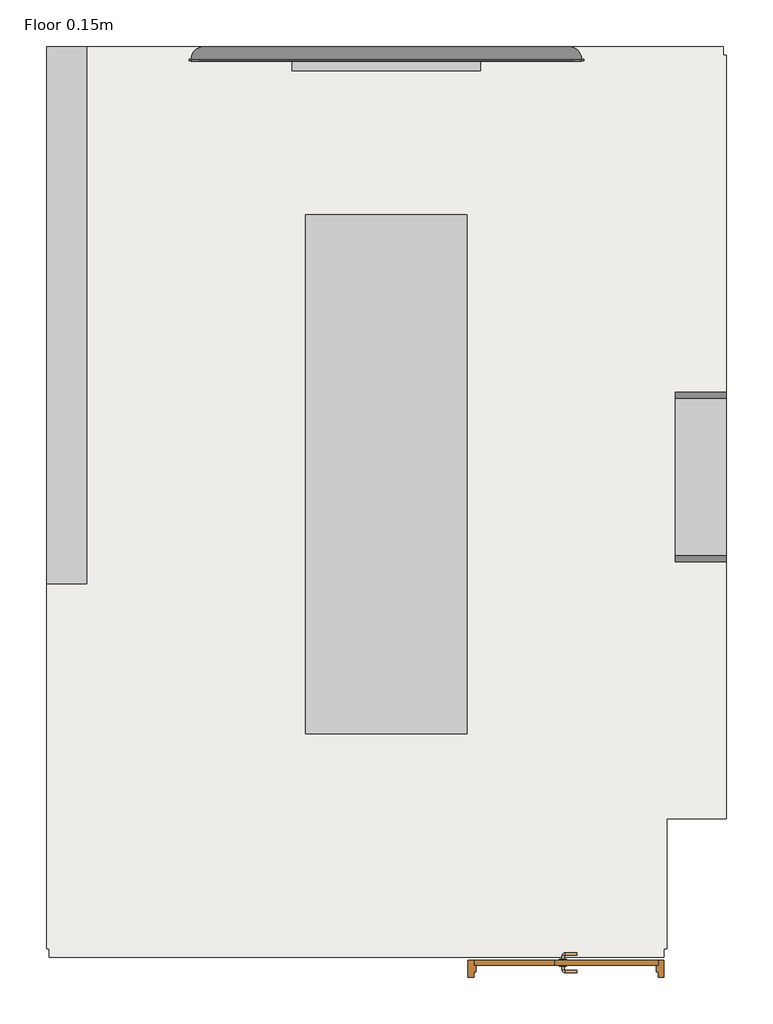
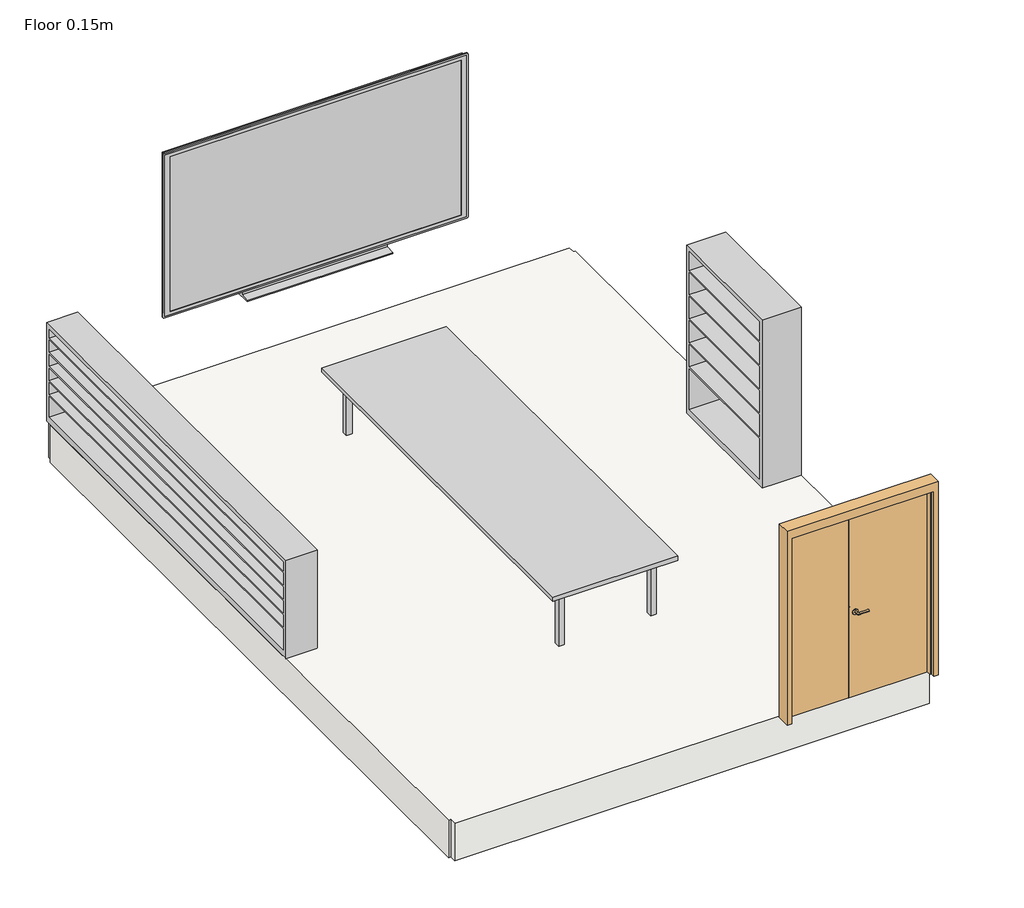
# One storey: 4 furniture elements, 1 door, 1 slab.
"""IFC4 building model written with IfcOpenShell, lengths in millimetres."""

import ifcopenshell
import ifcopenshell.guid

model = None  # the IFC model being written
_history = None  # IfcOwnerHistory: only IFC2X3 demands one
_inside = {}  # id of a spatial element -> (the spatial element, [elements in it])
_under = {}  # id of a project, library or spatial element -> (it, [spatial elements below it])
_declared = {}  # id of a project -> (the project, [libraries it declares])
_typed = {}  # id of a type object -> (the type object, [elements of that type])
_made_of = {}  # id of a material, layer set ... -> (it, [elements and type objects made of it])


def new_model(schema):
    """Start an empty IFC model of exactly this schema.

    Asked for "IFC4X3", IfcOpenShell would pick the latest addendum, in which some entities
    have other attributes; the version numbers below select the first issue.
    IFC2X3 requires an IfcOwnerHistory on every rooted entity: one is made here for all.
    """
    global model, _history
    if schema == "IFC4X3":
        model = ifcopenshell.file(schema_version=(4, 3, 0, 0))
    else:
        model = ifcopenshell.file(schema=schema)
    _inside.clear()
    _under.clear()
    _declared.clear()
    _typed.clear()
    _made_of.clear()
    _history = None
    if model.schema == "IFC2X3":
        org = make("IfcOrganization", Name="unknown")
        user = make(
            "IfcPersonAndOrganization",
            ThePerson=make("IfcPerson", FamilyName="unknown"),
            TheOrganization=org,
        )
        app = make(
            "IfcApplication",
            ApplicationDeveloper=org,
            Version="unknown",
            ApplicationFullName="unknown",
            ApplicationIdentifier="unknown",
        )
        _history = make(
            "IfcOwnerHistory",
            OwningUser=user,
            OwningApplication=app,
            ChangeAction="ADDED",
            CreationDate=0,
        )
    return model


def make(cls, **values):
    """One entity of the class cls with the attributes given. An attribute that is None is left unset."""
    return model.create_entity(
        cls, **{name: value for name, value in values.items() if value is not None}
    )


def rooted(cls, **values):
    """An entity with a GlobalId (a new one), such as an element, a storey or a relation."""
    return make(cls, GlobalId=ifcopenshell.guid.new(), OwnerHistory=_history, **values)


def si_unit(unit_type, name, prefix=None):
    """IfcSIUnit, for example si_unit("LENGTHUNIT", "METRE", prefix="MILLI")."""
    return make("IfcSIUnit", UnitType=unit_type, Prefix=prefix, Name=name)


def assignment(units):
    """IfcUnitAssignment: the units of a project."""
    return None if units is None else make("IfcUnitAssignment", Units=units)


def point(xyz):
    """IfcCartesianPoint."""
    return None if xyz is None else make("IfcCartesianPoint", Coordinates=xyz)


def direction(xyz):
    """IfcDirection."""
    return None if xyz is None else make("IfcDirection", DirectionRatios=xyz)


def frame(location, z_axis=None, x_axis=None):
    """IfcAxis2Placement3D, a coordinate frame: its origin and axes. An axis left out is left unset."""
    return make(
        "IfcAxis2Placement3D",
        Location=point(location),
        Axis=direction(z_axis),
        RefDirection=direction(x_axis),
    )


def frame_2d(location, x_axis=None):
    """IfcAxis2Placement2D, a coordinate frame in the plane: its origin and x axis."""
    return make(
        "IfcAxis2Placement2D", Location=point(location), RefDirection=direction(x_axis)
    )


def origin():
    """The frame at (0, 0, 0) with its axes left unset."""
    return frame((0.0, 0.0, 0.0))


def origin_with_axes():
    """The frame at (0, 0, 0) with the z axis (0, 0, 1) and the x axis (1, 0, 0) written out."""
    return frame((0.0, 0.0, 0.0), z_axis=(0.0, 0.0, 1.0), x_axis=(1.0, 0.0, 0.0))


def place(relative_to, where):
    """IfcLocalPlacement: puts the frame where relative to a parent placement (None: the world)."""
    return make(
        "IfcLocalPlacement", PlacementRelTo=relative_to, RelativePlacement=where
    )


def context(
    kind, dimensions, precision=None, world=None, true_north=None, identifier=None
):
    """IfcGeometricRepresentationContext, for example the 3D "Model" context."""
    return make(
        "IfcGeometricRepresentationContext",
        ContextIdentifier=identifier,
        ContextType=kind,
        CoordinateSpaceDimension=dimensions,
        Precision=precision,
        WorldCoordinateSystem=world,
        TrueNorth=true_north,
    )


def project(units=None, contexts=None):
    """IfcProject with its units and contexts."""
    return rooted(
        "IfcProject",
        Name="project",
        RepresentationContexts=contexts,
        UnitsInContext=assignment(units),
    )


def spatial(cls, under=None, at=None, **own):
    """A site, building, storey or space (cls), placed at a placement, below another one or the project."""
    s = rooted(cls, ObjectPlacement=at, **own)
    if under is not None:
        _under.setdefault(under.id(), (under, []))[1].append(s)
    return s


def polyline(points):
    """IfcPolyline through the points."""
    return make("IfcPolyline", Points=[point(p) for p in points])


def circle_curve(where, radius):
    """IfcCircle in the frame where."""
    return make("IfcCircle", Position=where, Radius=radius)


def ellipse_curve(where, semi_axis1, semi_axis2):
    """IfcEllipse in the frame where."""
    return make(
        "IfcEllipse", Position=where, SemiAxis1=semi_axis1, SemiAxis2=semi_axis2
    )


def trimmed(basis, trim1, trim2, sense, master):
    """IfcTrimmedCurve: the piece of a basis curve between two trims."""
    return make(
        "IfcTrimmedCurve",
        BasisCurve=basis,
        Trim1=trim1,
        Trim2=trim2,
        SenseAgreement=sense,
        MasterRepresentation=master,
    )


def segment(curve, same_sense, transition):
    """IfcCompositeCurveSegment."""
    return make(
        "IfcCompositeCurveSegment",
        Transition=transition,
        SameSense=same_sense,
        ParentCurve=curve,
    )


def composite_curve(segments, self_intersect=None):
    """IfcCompositeCurve: segments joined end to end."""
    return make("IfcCompositeCurve", Segments=segments, SelfIntersect=self_intersect)


def outline(outer, holes=None, kind="AREA"):
    """IfcArbitraryClosedProfileDef: a profile drawn as a closed curve; with holes, ...WithVoids."""
    if holes is None:
        return make("IfcArbitraryClosedProfileDef", ProfileType=kind, OuterCurve=outer)
    return make(
        "IfcArbitraryProfileDefWithVoids",
        ProfileType=kind,
        OuterCurve=outer,
        InnerCurves=holes,
    )


def extrude(swept, where, along, depth):
    """IfcExtrudedAreaSolid: the profile swept, set in the frame where, extruded along a direction by depth."""
    return make(
        "IfcExtrudedAreaSolid",
        SweptArea=swept,
        Position=where,
        ExtrudedDirection=direction(along),
        Depth=depth,
    )


def faces_of(points, faces, orient=None, outer=None):
    """IfcFace entities. A face is a list of loops; a loop is a list of indices into points, from 0.

    orient and outer hold one flag for each loop. By default every Orientation is true, the
    first loop of a face is its IfcFaceOuterBound and the others are IfcFaceBound.
    """
    made = []
    for i, loops in enumerate(faces):
        bounds = []
        for j, loop in enumerate(loops):
            is_outer = j == 0 if outer is None else outer[i][j]
            bounds.append(
                make(
                    "IfcFaceOuterBound" if is_outer else "IfcFaceBound",
                    Bound=make("IfcPolyLoop", Polygon=[points[k] for k in loop]),
                    Orientation=True if orient is None else orient[i][j],
                )
            )
        made.append(make("IfcFace", Bounds=bounds))
    return made


def faceted_brep(points, faces, orient=None, outer=None, voids=None):
    """IfcFacetedBrep: a solid bounded by flat faces; with voids (closed shells), ...WithVoids."""
    shared = [point(p) for p in points]
    hull = make("IfcClosedShell", CfsFaces=faces_of(shared, faces, orient, outer))
    if voids is None:
        return make("IfcFacetedBrep", Outer=hull)
    return make(
        "IfcFacetedBrepWithVoids",
        Outer=hull,
        Voids=[
            make(cls, CfsFaces=faces_of(shared, fs, o, b)) for cls, fs, o, b in voids
        ],
    )


def shape(context_of_items, identifier, shape_type, items):
    """IfcShapeRepresentation: the items that make up one representation, for example the "Body"."""
    return make(
        "IfcShapeRepresentation",
        ContextOfItems=context_of_items,
        RepresentationIdentifier=identifier,
        RepresentationType=shape_type,
        Items=items,
    )


def source(mapping_origin, context_of_items, identifier, shape_type, items):
    """IfcRepresentationMap: a shape defined once, which mapped items show again and again."""
    return make(
        "IfcRepresentationMap",
        MappingOrigin=mapping_origin,
        MappedRepresentation=shape(context_of_items, identifier, shape_type, items),
    )


def transform(
    local_origin,
    x_axis=None,
    y_axis=None,
    z_axis=None,
    scale=None,
    scale2=None,
    scale3=None,
    uniform=True,
):
    """IfcCartesianTransformationOperator3D, or its non-uniform kind. x_axis, y_axis, z_axis: its Axis1, 2, 3."""
    if uniform:
        return make(
            "IfcCartesianTransformationOperator3D",
            Axis1=direction(x_axis),
            Axis2=direction(y_axis),
            LocalOrigin=point(local_origin),
            Scale=scale,
            Axis3=direction(z_axis),
        )
    return make(
        "IfcCartesianTransformationOperator3DnonUniform",
        Axis1=direction(x_axis),
        Axis2=direction(y_axis),
        LocalOrigin=point(local_origin),
        Scale=scale,
        Axis3=direction(z_axis),
        Scale2=scale2,
        Scale3=scale3,
    )


def mapped(mapping_source, mapping_target):
    """IfcMappedItem: shows the shape of a source again, moved by a transform."""
    return make(
        "IfcMappedItem", MappingSource=mapping_source, MappingTarget=mapping_target
    )


def made_of(thing, what):
    """Note that an element or type object is made of a material, layer set ...; save() writes the relation."""
    if what is not None:
        _made_of.setdefault(what.id(), (what, []))[1].append(thing)
    return thing


def element(
    cls,
    number,
    at=None,
    inside=None,
    cuts=None,
    type_object=None,
    material=None,
    context=None,
    identifier="Body",
    shape_type=None,
    held_by="IfcProductDefinitionShape",
    body=None,
    shapes=None,
    **own,
):
    """One element of the class cls, such as IfcWall. Its Tag is "e" and its number.

    at: its placement. inside: the storey or other place that contains it. cuts: it is an
    opening in that element (IfcRelVoidsElement). A single representation is given by context,
    identifier, shape_type and body (its items); several are given by shapes. held_by: the class
    of the entity that holds the representations. save() writes the other relations.
    """
    e = rooted(cls, Tag="e%d" % number, ObjectPlacement=at, **own)
    if body is not None:
        shapes = [shape(context, identifier, shape_type, body)]
    if shapes is not None:
        e.Representation = make(held_by, Representations=shapes)
    if inside is not None:
        _inside.setdefault(inside.id(), (inside, []))[1].append(e)
    if cuts is not None:
        rooted(
            "IfcRelVoidsElement", RelatingBuildingElement=cuts, RelatedOpeningElement=e
        )
    if type_object is not None:
        _typed.setdefault(type_object.id(), (type_object, []))[1].append(e)
    return made_of(e, material)


def aggregate(whole, parts):
    """IfcRelAggregates: a whole, such as a stair, and the parts it consists of."""
    return rooted("IfcRelAggregates", RelatingObject=whole, RelatedObjects=parts)


def save(model, path):
    """Write the relations noted so far, then the file.

    IfcRelAggregates (storeys below a building ...), IfcRelContainedInSpatialStructure (elements
    in a storey), IfcRelDefinesByType, IfcRelAssociatesMaterial and IfcRelDeclares: one each for
    every whole, place, type object, material and project.
    """
    for whole, parts in _under.values():
        aggregate(whole, parts)
    for where, things in _inside.values():
        rooted(
            "IfcRelContainedInSpatialStructure",
            RelatedElements=things,
            RelatingStructure=where,
        )
    for kind, things in _typed.values():
        rooted("IfcRelDefinesByType", RelatedObjects=things, RelatingType=kind)
    for what, things in _made_of.values():
        rooted("IfcRelAssociatesMaterial", RelatedObjects=things, RelatingMaterial=what)
    for by, libraries in _declared.values():
        rooted("IfcRelDeclares", RelatingContext=by, RelatedDefinitions=libraries)
    model.write(path)


def plane_surface(at):
    """IfcPlane: the flat surface through the origin of the frame at, square to its z axis."""
    return make("IfcPlane", Position=at)


def cylinder_surface(at, radius):
    """IfcCylindricalSurface: all points at the distance radius from the z axis of the frame at."""
    return make("IfcCylindricalSurface", Position=at, Radius=radius)


def revolved_surface(curve, axis_point, axis_direction):
    """IfcSurfaceOfRevolution: the curve turned about the line through axis_point along axis_direction."""
    return make(
        "IfcSurfaceOfRevolution",
        SweptCurve=make("IfcArbitraryOpenProfileDef", ProfileType="CURVE", Curve=curve),
        AxisPosition=make("IfcAxis1Placement", Location=point(axis_point), Axis=direction(axis_direction)),
    )


def advanced_brep(points, edges, surfaces, faces):
    """IfcAdvancedBrep: a solid bounded by faces that lie on surfaces and meet in shared edges.

    An edge is (start, end): straight between two places in points (the first is 0);
    or (start, end, curve); or (start, end, curve, False) where it runs against its curve.
    A face is (place in surfaces, loops), or (place, loops, False) where it looks against
    its surface's normal. A loop lists edges by number (the first is 1), with a minus sign
    where the edge is run from its end to its start. The first loop is the outer one.
    """
    corners = [point(p) for p in points]
    vertices = [make("IfcVertexPoint", VertexGeometry=c) for c in corners]
    made = []
    for start, end, *more in edges:
        made.append(
            make(
                "IfcEdgeCurve",
                EdgeStart=vertices[start],
                EdgeEnd=vertices[end],
                EdgeGeometry=more[0] if more else make("IfcPolyline", Points=[corners[start], corners[end]]),
                SameSense=more[1] if len(more) > 1 else True,
            )
        )
    hull = []
    for where, loops, *sense in faces:
        bounds = []
        for j, loop in enumerate(loops):
            ring = [make("IfcOrientedEdge", EdgeElement=made[abs(k) - 1], Orientation=k > 0) for k in loop]
            bounds.append(
                make(
                    "IfcFaceOuterBound" if j == 0 else "IfcFaceBound",
                    Bound=make("IfcEdgeLoop", EdgeList=ring),
                    Orientation=True,
                )
            )
        hull.append(make("IfcAdvancedFace", Bounds=bounds, FaceSurface=surfaces[where], SameSense=sense[0] if sense else True))
    return make("IfcAdvancedBrep", Outer=make("IfcClosedShell", CfsFaces=hull))


def m_door_passage_uneven_flush_1600_x_2200_848efb9c(model_context):
    return source(origin(), model_context, "Body", "SolidModel", [
        advanced_brep(
        [(34.59375, 9.15, 1000.0), (14.59375, 9.15, 1000.0), (14.59375, 39.15, 1000.0), (34.59375, 39.15, 1000.0), (9.59375, 44.15, 1000.0), (9.59375, 64.15, 1000.0), (-95.40625, 64.15, 1000.0), (-95.40625, 44.15, 1000.0)],
        [
            (0, 1, circle_curve(frame((24.59375, 9.15, 1000.0), z_axis=(0.0, -1.0, 0.0), x_axis=(-1.0, 0.0, 0.0)), 10.0)),
            (1, 0, circle_curve(frame((24.59375, 9.15, 1000.0), z_axis=(0.0, -1.0, 0.0), x_axis=(-1.0, 0.0, 0.0)), 10.0)),
            (1, 2),
            (2, 3, circle_curve(frame((24.59375, 39.15, 1000.0), z_axis=(0.0, -1.0, 0.0), x_axis=(-1.0, 0.0, 0.0)), 10.0)),
            (3, 0),
            (3, 2, circle_curve(frame((24.59375, 39.15, 1000.0), z_axis=(0.0, -1.0, 0.0), x_axis=(-1.0, 0.0, 0.0)), 10.0)),
            (4, 5, circle_curve(frame((9.59375, 54.15, 1000.0), z_axis=(1.0, 0.0, 0.0), x_axis=(0.0, -1.0, 0.0)), 10.0)),
            (5, 3, circle_curve(frame((9.59375, 39.15, 1000.0), z_axis=(0.0, 0.0, -1.0), x_axis=(1.0, 0.0, 0.0)), 25.0)),
            (2, 4, circle_curve(frame((9.59375, 39.15, 1000.0), z_axis=(0.0, 0.0, 1.0), x_axis=(1.0, 0.0, 0.0)), 5.0)),
            (5, 4, circle_curve(frame((9.59375, 54.15, 1000.0), z_axis=(1.0, 0.0, 0.0), x_axis=(0.0, -1.0, 0.0)), 10.0)),
            (6, 7, circle_curve(frame((-95.40625, 54.15, 1000.0), z_axis=(-1.0, 0.0, 0.0), x_axis=(0.0, -1.0, 0.0)), 10.0)),
            (7, 6, circle_curve(frame((-95.40625, 54.15, 1000.0), z_axis=(-1.0, 0.0, 0.0), x_axis=(0.0, -1.0, 0.0)), 10.0)),
            (4, 7),
            (6, 5),
        ],
        [
            plane_surface(frame((24.59375, 9.15, 1000.0), z_axis=(0.0, -1.0, 0.0), x_axis=(0.0, 0.0, 1.0))),
            cylinder_surface(frame((24.59375, 9.15, 1000.0), z_axis=(0.0, -1.0, 0.0), x_axis=(-1.0, 0.0, 0.0)), 10.0),
            revolved_surface(trimmed(ellipse_curve(frame((24.59375, 39.15, 1000.0), z_axis=(0.0, 1.0, 0.0), x_axis=(-1.0, 0.0, 0.0)), 10.0, 10.0), [point((34.59375, 39.15, 1000.0))], [point((14.59375, 39.15, 1000.0))], True, "CARTESIAN"), (9.59375, 39.15, 1000.0), (0.0, 0.0, -1.0)),
            revolved_surface(trimmed(ellipse_curve(frame((24.59375, 39.15, 1000.0), z_axis=(0.0, 1.0, 0.0), x_axis=(-1.0, 0.0, 0.0)), 10.0, 10.0), [point((14.59375, 39.15, 1000.0))], [point((34.59375, 39.15, 1000.0))], True, "CARTESIAN"), (9.59375, 39.15, 1000.0), (0.0, 0.0, -1.0)),
            plane_surface(frame((-95.40625, 54.15, 1000.0), z_axis=(-1.0, 0.0, 0.0), x_axis=(0.0, 0.0, 1.0))),
            cylinder_surface(frame((9.59375, 54.15, 1000.0), z_axis=(1.0, 0.0, 0.0), x_axis=(0.0, -1.0, 0.0)), 10.0),
        ],
        [
            (0, [[1, 2]]),
            (1, [[3, 4, 5, -2]]),
            (1, [[-5, 6, -3, -1]]),
            (2, [[7, 8, -4, 9]]),
            (3, [[10, -9, -6, -8]]),
            (4, [[11, 12]]),
            (5, [[13, -11, 14, -7]]),
            (5, [[-14, -12, -13, -10]]),
        ],
    ),
        extrude(outline(composite_curve([segment(trimmed(circle_curve(frame_2d((1000.0, 27.09375)), 30.0), [point((1000.0, 57.09375))], [point((1000.0, -2.90625))], False, "CARTESIAN"), True, "CONTINUOUS"), segment(trimmed(circle_curve(frame_2d((1000.0, 27.09375)), 30.0), [point((1000.0, -2.90625))], [point((1000.0, 57.09375))], False, "CARTESIAN"), True, "CONTINUOUS")], self_intersect=False)), frame((0.0, 1.15, 0.0), z_axis=(0.0, 1.0, 0.0), x_axis=(0.0, 0.0, 1.0)), (0.0, 0.0, 1.0), 8.0),
        advanced_brep(
        [(34.59375, -51.85, 1000.0), (14.59375, -51.85, 1000.0), (34.59375, -81.85, 1000.0), (14.59375, -81.85, 1000.0), (9.59375, -86.85, 1000.0), (9.59375, -106.85, 1000.0), (-95.40625, -106.85, 1000.0), (-95.40625, -86.85, 1000.0)],
        [
            (0, 1, circle_curve(frame((24.59375, -51.85, 1000.0), z_axis=(0.0, 1.0, 0.0), x_axis=(-1.0, 0.0, 0.0)), 10.0)),
            (1, 0, circle_curve(frame((24.59375, -51.85, 1000.0), z_axis=(0.0, 1.0, 0.0), x_axis=(-1.0, 0.0, 0.0)), 10.0)),
            (0, 2),
            (2, 3, circle_curve(frame((24.59375, -81.85, 1000.0), z_axis=(0.0, 1.0, 0.0), x_axis=(-1.0, 0.0, 0.0)), 10.0)),
            (3, 1),
            (3, 2, circle_curve(frame((24.59375, -81.85, 1000.0), z_axis=(0.0, 1.0, 0.0), x_axis=(-1.0, 0.0, 0.0)), 10.0)),
            (4, 3, circle_curve(frame((9.59375, -81.85, 1000.0), z_axis=(0.0, 0.0, 1.0), x_axis=(1.0, 0.0, 0.0)), 5.0)),
            (2, 5, circle_curve(frame((9.59375, -81.85, 1000.0), z_axis=(0.0, 0.0, -1.0), x_axis=(1.0, 0.0, 0.0)), 25.0)),
            (5, 4, circle_curve(frame((9.59375, -96.85, 1000.0), z_axis=(1.0, 0.0, 0.0), x_axis=(0.0, 1.0, 0.0)), 10.0)),
            (4, 5, circle_curve(frame((9.59375, -96.85, 1000.0), z_axis=(1.0, 0.0, 0.0), x_axis=(0.0, 1.0, 0.0)), 10.0)),
            (6, 7, circle_curve(frame((-95.40625, -96.85, 1000.0), z_axis=(-1.0, 0.0, 0.0), x_axis=(0.0, 1.0, 0.0)), 10.0)),
            (7, 6, circle_curve(frame((-95.40625, -96.85, 1000.0), z_axis=(-1.0, 0.0, 0.0), x_axis=(0.0, 1.0, 0.0)), 10.0)),
            (5, 6),
            (7, 4),
        ],
        [
            plane_surface(frame((24.59375, -51.85, 1000.0), z_axis=(0.0, 1.0, 0.0), x_axis=(0.0, 0.0, 1.0))),
            cylinder_surface(frame((24.59375, -51.85, 1000.0), z_axis=(0.0, 1.0, 0.0), x_axis=(-1.0, 0.0, 0.0)), 10.0),
            revolved_surface(trimmed(ellipse_curve(frame((24.59375, -81.85, 1000.0), z_axis=(0.0, 1.0, 0.0), x_axis=(-1.0, 0.0, 0.0)), 10.0, 10.0), [point((34.59375, -81.85, 1000.0))], [point((14.59375, -81.85, 1000.0))], True, "CARTESIAN"), (9.59375, -81.85, 1000.0), (0.0, 0.0, -1.0)),
            revolved_surface(trimmed(ellipse_curve(frame((24.59375, -81.85, 1000.0), z_axis=(0.0, 1.0, 0.0), x_axis=(-1.0, 0.0, 0.0)), 10.0, 10.0), [point((14.59375, -81.85, 1000.0))], [point((34.59375, -81.85, 1000.0))], True, "CARTESIAN"), (9.59375, -81.85, 1000.0), (0.0, 0.0, -1.0)),
            plane_surface(frame((-95.40625, -96.85, 1000.0), z_axis=(-1.0, 0.0, 0.0), x_axis=(0.0, 0.0, 1.0))),
            cylinder_surface(frame((9.59375, -96.85, 1000.0), z_axis=(1.0, 0.0, 0.0), x_axis=(0.0, 1.0, 0.0)), 10.0),
        ],
        [
            (0, [[1, 2]]),
            (1, [[-1, 3, 4, 5]]),
            (1, [[-2, -5, 6, -3]]),
            (2, [[7, -4, 8, 9]]),
            (3, [[-8, -6, -7, 10]]),
            (4, [[11, 12]]),
            (5, [[-9, 13, -12, 14]]),
            (5, [[-10, -14, -11, -13]]),
        ],
    ),
        extrude(outline(composite_curve([segment(trimmed(circle_curve(frame_2d((1000.0, 27.09375)), 30.0), [point((1000.0, 57.09375))], [point((1000.0, -2.90625))], False, "CARTESIAN"), True, "CONTINUOUS"), segment(trimmed(circle_curve(frame_2d((1000.0, 27.09375)), 30.0), [point((1000.0, -2.90625))], [point((1000.0, 57.09375))], False, "CARTESIAN"), True, "CONTINUOUS")], self_intersect=False)), frame((0.0, -51.85, 0.0), z_axis=(0.0, 1.0, 0.0), x_axis=(0.0, 0.0, 1.0)), (0.0, 0.0, 1.0), 8.0),
        extrude(outline(polyline([(98.4, 1.15), (98.4, -43.85), (-800.0, -43.85), (-800.0, 1.15), (98.4, 1.15)])), origin_with_axes(), (0.0, 0.0, 1.0), 2200.0),
        faceted_brep([(800.0, 5.9125, 0.0), (784.125, 5.9125, 0.0), (784.125, 56.9375, 0.0), (800.0, 56.9375, 0.0), (800.0, 106.15, 0.0), (850.0, 106.15, 0.0), (850.0, -43.85, 0.0), (800.0, -43.85, 0.0), (800.0, -43.85, 2200.0), (800.0, 5.9125, 2200.0), (850.0, -43.85, 2300.0), (-850.0, -43.85, 2300.0), (-850.0, -43.85, 0.0), (-800.0, -43.85, 0.0), (-800.0, -43.85, 2200.0), (850.0, 106.15, 2300.0), (800.0, 106.15, 2200.0), (-800.0, 106.15, 2200.0), (-800.0, 106.15, 0.0), (-850.0, 106.15, 0.0), (-850.0, 106.15, 2300.0), (800.0, 56.9375, 2200.0), (784.125, 56.9375, 2184.125), (-784.125, 56.9375, 2184.125), (-784.125, 56.9375, 0.0), (-800.0, 56.9375, 0.0), (-800.0, 56.9375, 2200.0), (784.125, 5.9125, 2184.125), (-800.0, 5.9125, 2200.0), (-800.0, 5.9125, 0.0), (-784.125, 5.9125, 0.0), (-784.125, 5.9125, 2184.125)], [[[0, 1, 2, 3, 4, 5, 6, 7]], [[7, 8, 9, 0]], [[6, 10, 11, 12, 13, 14, 8, 7]], [[5, 15, 10, 6]], [[4, 16, 17, 18, 19, 20, 15, 5]], [[3, 21, 16, 4]], [[2, 22, 23, 24, 25, 26, 21, 3]], [[1, 27, 22, 2]], [[0, 9, 28, 29, 30, 31, 27, 1]], [[8, 14, 28, 9]], [[16, 21, 26, 17]], [[22, 27, 31, 23]], [[12, 19, 18, 25, 24, 30, 29, 13]], [[13, 29, 28, 14]], [[11, 20, 19, 12]], [[17, 26, 25, 18]], [[23, 31, 30, 24]], [[15, 20, 11, 10]]]),
        extrude(outline(polyline([(800.0, 1.15), (800.0, -43.85), (101.6, -43.85), (101.6, 1.15), (800.0, 1.15)])), origin_with_axes(), (0.0, 0.0, 1.0), 2200.0),
    ])


def furniture_0810mm_1eea789d(model_context):
    return source(origin(), model_context, "Body", "SolidModel", [
        advanced_brep(
        [(-1698.1126034, -51.4613764, 80.0), (1690.2235751, -51.4613764, 80.0), (1690.2235751, -51.4613764, 1998.6077952), (-1698.1126034, -51.4613764, 1998.6077952), (1580.2235751, 58.5386236, 80.0), (-1588.1126034, 58.5386236, 80.0), (-1588.1126034, 58.5386236, 1888.6077952), (1580.2235751, 58.5386236, 1888.6077952)],
        [
            (0, 1),
            (1, 2),
            (2, 3),
            (3, 0),
            (4, 5),
            (5, 6),
            (6, 7),
            (7, 4),
            (0, 5, circle_curve(frame((-1588.1126034, -51.4613764, 80.0), z_axis=(0.0, 0.0, -1.0), x_axis=(-1.0, 0.0, 0.0)), 110.0)),
            (4, 1, circle_curve(frame((1580.2235751, -51.4613764, 80.0), z_axis=(0.0, 0.0, -1.0), x_axis=(1.0, 0.0, 0.0)), 110.0)),
            (7, 2, ellipse_curve(frame((1580.2235751, -51.4613764, 1888.6077952), z_axis=(0.7071067811865475, 0.0, -0.7071067811865475), x_axis=(0.7071067811865474, 0.0, 0.7071067811865476)), 155.5634919, 110.0)),
            (6, 3, ellipse_curve(frame((-1588.1126034, -51.4613764, 1888.6077952), z_axis=(0.7071067811865475, 0.0, 0.7071067811865475), x_axis=(-0.7071067811865476, 0.0, 0.7071067811865474)), 155.5634919, 110.0)),
        ],
        [
            plane_surface(frame((-1698.1126034, -51.4613764, 1998.6077952), z_axis=(0.0, -1.0, 0.0), x_axis=(-1.0, 0.0, 0.0))),
            plane_surface(frame((-1698.1126034, 58.5386236, 1998.6077952), z_axis=(0.0, 1.0, 0.0), x_axis=(1.0, 0.0, 0.0))),
            plane_surface(frame((-1698.1126034, -51.4613764, 80.0), z_axis=(0.0, 0.0, -1.0), x_axis=(0.0, 1.0, 0.0))),
            cylinder_surface(frame((1580.2235751, -51.4613764, 80.0), z_axis=(0.0, 0.0, 1.0), x_axis=(1.0, 0.0, 0.0)), 110.0),
            cylinder_surface(frame((1690.2235751, -51.4613764, 1888.6077952), z_axis=(-1.0, 0.0, 0.0), x_axis=(0.0, 0.0, 1.0)), 110.0),
            cylinder_surface(frame((-1588.1126034, -51.4613764, 1998.6077952), z_axis=(0.0, 0.0, -1.0), x_axis=(-1.0, 0.0, 0.0)), 110.0),
        ],
        [
            (0, [[1, 2, 3, 4]]),
            (1, [[5, 6, 7, 8]]),
            (2, [[-1, 9, -5, 10]]),
            (3, [[11, -2, -10, -8]]),
            (4, [[-11, -7, 12, -3]]),
            (5, [[-12, -6, -9, -4]]),
        ],
    ),
        extrude(outline(composite_curve([segment(polyline([(2018.6077952, 1695.2235751), (2018.6077952, -1703.1126034)]), True, "CONTINUOUS"), segment(trimmed(circle_curve(frame_2d((2003.6077952, -1703.1126034)), 15.0), [point((2018.6077952, -1703.1126034))], [point((2003.6077952, -1718.1126034))], False, "CARTESIAN"), True, "CONTINUOUS"), segment(polyline([(2003.6077952, -1718.1126034), (75.0, -1718.1126034)]), True, "CONTINUOUS"), segment(trimmed(circle_curve(frame_2d((75.0, -1703.1126034)), 15.0), [point((75.0, -1718.1126034))], [point((60.0, -1703.1126034))], False, "CARTESIAN"), True, "CONTINUOUS"), segment(polyline([(60.0, -1703.1126034), (60.0, 1695.2235751)]), True, "CONTINUOUS"), segment(trimmed(circle_curve(frame_2d((75.0, 1695.2235751)), 15.0), [point((60.0, 1695.2235751))], [point((75.0, 1710.2235751))], False, "CARTESIAN"), True, "CONTINUOUS"), segment(polyline([(75.0, 1710.2235751), (2003.6077952, 1710.2235751)]), True, "CONTINUOUS"), segment(trimmed(circle_curve(frame_2d((2003.6077952, 1695.2235751)), 15.0), [point((2003.6077952, 1710.2235751))], [point((2018.6077952, 1695.2235751))], False, "CARTESIAN"), True, "CONTINUOUS")], self_intersect=False), holes=[polyline([(1998.6077952, 1690.2235751), (80.0, 1690.2235751), (80.0, -1698.1126034), (1998.6077952, -1698.1126034), (1998.6077952, 1690.2235751)])]), frame((0.0, -66.4613764, 0.0), z_axis=(0.0, 1.0, 0.0), x_axis=(0.0, 0.0, 1.0)), (0.0, 0.0, 1.0), 15.0),
        faceted_brep([(1690.2235751, -69.4613764, 1998.6077952), (-1698.1126034, -69.4613764, 1998.6077952), (-1698.1126034, -69.4613764, 80.0), (1690.2235751, -69.4613764, 80.0), (-1638.1126034, -69.4613764, 1958.6077952), (1630.2235751, -69.4613764, 1958.6077952), (1630.2235751, -69.4613764, 120.0), (-1638.1126034, -69.4613764, 120.0), (1690.2235751, -51.4613764, 1998.6077952), (1690.2235751, -51.4613764, 80.0), (-1698.1126034, -51.4613764, 80.0), (-1698.1126034, -51.4613764, 1998.6077952), (-1638.1126034, -66.4613764, 1958.6077952), (-1638.1126034, -66.4613764, 120.0), (1630.2235751, -66.4613764, 120.0), (1630.2235751, -66.4613764, 1958.6077952)], [[[0, 1, 2, 3], [4, 5, 6, 7]], [[8, 9, 10, 11]], [[1, 0, 8, 11]], [[2, 1, 11, 10]], [[3, 2, 10, 9]], [[0, 3, 9, 8]], [[12, 13, 14, 15]], [[12, 15, 5, 4]], [[15, 14, 6, 5]], [[14, 13, 7, 6]], [[13, 12, 4, 7]]]),
        extrude(outline(polyline([(-51.4613764, 80.0), (-1.4613764, 80.0), (48.5386236, 0.0), (-151.4613764, 0.0), (-151.4613764, 10.0), (-51.4613764, 20.0), (-51.4613764, 80.0)])), frame((-821.0285588, 0.0, 0.0), z_axis=(1.0, 0.0, 0.0), x_axis=(0.0, 1.0, 0.0)), (0.0, 0.0, 1.0), 1634.1680892),
    ])


def m_shelving_left_2_f9164daf(model_context):
    return source(origin(), model_context, "Body", "SweptSolid", [
        extrude(outline(polyline([(0.0, 2330.0), (1170.0, 2330.0), (1170.0, -2330.0), (0.0, -2330.0), (0.0, 2330.0)]), holes=[polyline([(1119.2, 2279.2), (1015.5571429, 2279.2), (1015.5571429, -2279.2), (1119.2, -2279.2), (1119.2, 2279.2)]), polyline([(76.2, 2279.2), (76.2, -2279.2), (321.5857143, -2279.2), (321.5857143, 2279.2), (76.2, 2279.2)]), polyline([(681.2714286, -2279.2), (823.0142857, -2279.2), (823.0142857, 2279.2), (681.2714286, 2279.2), (681.2714286, -2279.2)]), polyline([(990.1571429, 2279.2), (848.4142857, 2279.2), (848.4142857, -2279.2), (990.1571429, -2279.2), (990.1571429, 2279.2)]), polyline([(655.8714286, 2279.2), (514.1285714, 2279.2), (514.1285714, -2279.2), (655.8714286, -2279.2), (655.8714286, 2279.2)]), polyline([(488.7285714, 2279.2), (346.9857143, 2279.2), (346.9857143, -2279.2), (488.7285714, -2279.2), (488.7285714, 2279.2)])]), frame((0.0, -479.8, 0.0), z_axis=(0.0, 1.0, 0.0), x_axis=(0.0, 0.0, 1.0)), (0.0, 0.0, 1.0), 350.0),
    ])


def m_shelving_right_232c7dd4(model_context):
    return source(origin(), model_context, "Body", "SweptSolid", [
        extrude(outline(polyline([(0.0, 735.0), (2000.0, 735.0), (2000.0, -735.0), (0.0, -735.0), (0.0, 735.0)]), holes=[polyline([(1949.2, 684.2), (1726.9857143, 684.2), (1726.9857143, -684.2), (1949.2, -684.2), (1949.2, 684.2)]), polyline([(76.2, 684.2), (76.2, -684.2), (558.7285714, -684.2), (558.7285714, 684.2), (76.2, 684.2)]), polyline([(1155.5571429, -684.2), (1415.8714286, -684.2), (1415.8714286, 684.2), (1155.5571429, 684.2), (1155.5571429, -684.2)]), polyline([(1701.5857143, 684.2), (1441.2714286, 684.2), (1441.2714286, -684.2), (1701.5857143, -684.2), (1701.5857143, 684.2)]), polyline([(1130.1571429, 684.2), (869.8428571, 684.2), (869.8428571, -684.2), (1130.1571429, -684.2), (1130.1571429, 684.2)]), polyline([(844.4428571, 684.2), (584.1285714, 684.2), (584.1285714, -684.2), (844.4428571, -684.2), (844.4428571, 684.2)])]), frame((0.0, -524.8, 0.0), z_axis=(0.0, 1.0, 0.0), x_axis=(0.0, 0.0, 1.0)), (0.0, 0.0, 1.0), 440.0),
    ])


def m_table_rectangular_table_5a2d8c47(model_context):
    return source(origin(), model_context, "Body", "SweptSolid", [
        extrude(outline(polyline([(-2034.1, 547.6), (-2034.1, 484.1), (-2097.6, 484.1), (-2097.6, 547.6), (-2034.1, 547.6)])), origin_with_axes(), (0.0, 0.0, 1.0), 679.2),
        extrude(outline(polyline([(2034.1, 547.6), (2097.6, 547.6), (2097.6, 484.1), (2034.1, 484.1), (2034.1, 547.6)])), origin_with_axes(), (0.0, 0.0, 1.0), 679.2),
        extrude(outline(polyline([(-2034.1, -547.6), (-2097.6, -547.6), (-2097.6, -484.1), (-2034.1, -484.1), (-2034.1, -547.6)])), origin_with_axes(), (0.0, 0.0, 1.0), 679.2),
        extrude(outline(polyline([(2034.1, -547.6), (2034.1, -484.1), (2097.6, -484.1), (2097.6, -547.6), (2034.1, -547.6)])), origin_with_axes(), (0.0, 0.0, 1.0), 679.2),
        extrude(outline(polyline([(2250.0, 700.0), (2250.0, -700.0), (-2250.0, -700.0), (-2250.0, 700.0), (2250.0, 700.0)])), frame((0.0, 0.0, 679.2), z_axis=(0.0, 0.0, 1.0), x_axis=(1.0, 0.0, 0.0)), (0.0, 0.0, 1.0), 50.8),
        extrude(outline(polyline([(2034.1, 509.5), (2034.1, 484.1), (-2034.1, 484.1), (-2034.1, 509.5), (2034.1, 509.5)])), frame((0.0, 0.0, 577.6), z_axis=(0.0, 0.0, 1.0), x_axis=(1.0, 0.0, 0.0)), (0.0, 0.0, 1.0), 101.6),
        extrude(outline(polyline([(2034.1, -509.5), (-2034.1, -509.5), (-2034.1, -484.1), (2034.1, -484.1), (2034.1, -509.5)])), frame((0.0, 0.0, 577.6), z_axis=(0.0, 0.0, 1.0), x_axis=(1.0, 0.0, 0.0)), (0.0, 0.0, 1.0), 101.6),
        extrude(outline(polyline([(-2046.8, -484.1), (-2072.2, -484.1), (-2072.2, 484.1), (-2046.8, 484.1), (-2046.8, -484.1)])), frame((0.0, 0.0, 577.6), z_axis=(0.0, 0.0, 1.0), x_axis=(1.0, 0.0, 0.0)), (0.0, 0.0, 1.0), 101.6),
        extrude(outline(polyline([(2046.8, -484.1), (2046.8, 484.1), (2072.2, 484.1), (2072.2, -484.1), (2046.8, -484.1)])), frame((0.0, 0.0, 577.6), z_axis=(0.0, 0.0, 1.0), x_axis=(1.0, 0.0, 0.0)), (0.0, 0.0, 1.0), 101.6),
    ])


model = new_model("IFC4")

# Units and contexts
model_context = context("Model", 3, world=origin())
ifc_project = project(units=[si_unit("LENGTHUNIT", "METRE", prefix="MILLI")], contexts=[model_context])

# Site, building, storey
site = spatial("IfcSite", under=ifc_project)
building = spatial("IfcBuilding", under=site)
storey = spatial("IfcBuildingStorey", under=building, Name="Floor 0.15m", Elevation=150.0)

# Door
placement = place(None, origin())
m_door_passage_uneven_flush_1600_x_2200_shape = m_door_passage_uneven_flush_1600_x_2200_848efb9c(model_context)
element("IfcDoor", 1, ObjectType="M_Door-Passage-Uneven-Flush : 1600 X 2200", at=placement, inside=storey, context=model_context, shape_type="MappedRepresentation", body=[
    mapped(m_door_passage_uneven_flush_1600_x_2200_shape, transform((1406.2835652, -4036.1029692, 150.0), x_axis=(-1.0, 0.0, 0.0), y_axis=(0.0, -1.0, 0.0), z_axis=(0.0, 0.0, 1.0))),
])

# Furniture
furniture_0810mm_shape = furniture_0810mm_1eea789d(model_context)
element("IfcFurniture", 2, ObjectType="M_TV - Flat Screen : 0810mm", at=placement, inside=storey, context=model_context, shape_type="MappedRepresentation", body=[
    mapped(furniture_0810mm_shape, transform((-149.7719206, 3874.2084071, 950.0), x_axis=(1.0, 0.0, 0.0), y_axis=(0.0, 1.0, 0.0), z_axis=(0.0, 0.0, 1.0))),
])
m_shelving_left_2_shape = m_shelving_left_2_f9164daf(model_context)
element("IfcFurniture", 3, ObjectType="M_Shelving : LEFT_2", at=placement, inside=storey, context=model_context, shape_type="MappedRepresentation", body=[
    mapped(m_shelving_left_2_shape, transform((-3233.5164348, 1602.7470308, 150.0), x_axis=(0.0, 1.0, 0.0), y_axis=(-1.0, 0.0, 0.0), z_axis=(0.0, 0.0, 1.0))),
])
m_shelving_right_shape = m_shelving_right_232c7dd4(model_context)
element("IfcFurniture", 4, ObjectType="M_Shelving : RIGHT", at=placement, inside=storey, context=model_context, shape_type="MappedRepresentation", body=[
    mapped(m_shelving_right_shape, transform((2271.4835652, 197.7470308, 150.0), x_axis=(0.0, 1.0, 0.0), y_axis=(-1.0, 0.0, 0.0), z_axis=(0.0, 0.0, 1.0))),
])
m_table_rectangular_table_shape = m_table_rectangular_table_5a2d8c47(model_context)
element("IfcFurniture", 5, ObjectType="M_Table-Rectangular : TABLE", at=placement, inside=storey, context=model_context, shape_type="MappedRepresentation", body=[
    mapped(m_table_rectangular_table_shape, transform((-153.7164348, 222.7470308, 150.0), x_axis=(0.0, 1.0, 0.0), y_axis=(-1.0, 0.0, 0.0), z_axis=(0.0, 0.0, 1.0))),
])

# Slab
element("IfcSlab", 6, ObjectType="FLOOR", at=placement, inside=storey, context=model_context, shape_type="SweptSolid", body=[
    extrude(outline(polyline([(-3078.7164348, -3892.2529692), (-3103.7164348, -3892.2529692), (-3103.7164348, 3857.7470308), (-3078.7164348, 3857.7470308), (-3078.7164348, 3932.7470308), (2771.2835652, 3932.7470308), (2771.2835652, 3857.7470308), (2796.2835652, 3857.7470308), (2796.2835652, -2767.2529692), (2281.2835652, -2767.2529692), (2281.2835652, -3892.2529692), (2256.2835652, -3892.2529692), (2256.2835652, -3967.2529692), (-3078.7164348, -3967.2529692), (-3078.7164348, -3892.2529692)])), frame((0.0, 0.0, -295.0), z_axis=(0.0, 0.0, 1.0), x_axis=(1.0, 0.0, 0.0)), (0.0, 0.0, 1.0), 445.0),
])

save(model, "model.ifc")

# Revit data of these elements
# Type "M_Door-Passage-Uneven-Flush : 1600 X 2200"
#   Type Mark = "50"
#   Assembly Code = "C1020300"
#   Analytic Construction = "Wooden"
#   Width Large Panel = 900 mm
#   W = 700 mm
#   Thickness = 45 mm
#   Thermal Resistance (R) = 0.455703 (m²·K)/W
#   Swing Angle [instance default] = 90.00°
#   Strike Height = 1000 mm
#   Rough Width [instance default] = 1700 mm
#   Rough Height [instance default] = 2300 mm
#   Masonry Frame Opening Height [instance default] = 100 mm
#   Masonry Frame Opening Width [instance default] = 100 mm
#   Inset Calculation [instance default] = 105 mm
#   Masonry Inset [instance default] = 25 mm
#   Height = 2200 mm
#   Width = 1600 mm
#   Heat Transfer Coefficient (U) = 2.19465 W/(m²·K)
#   Masonry Frame Depth = 150 mm
#   Masonry Frame [instance default] = yes
#   Dry Wall Frame [instance default] = no
#   Panel Material = Wood - Birch
#   Frame Material = Metal - Paint Finish - Grey
#   Door Handle Material = Aluminum
#   Visual Light Transmittance = 0
#   Solar Heat Gain Coefficient = 0
#   Wall Closure = (empty or 0)
#   Function = (empty or 0)
# Type "M_TV - Flat Screen : 0810mm"
#   SinAng = 0.49 mm
#   L = 3268.336 mm
#   H = 1838.608 mm
#   Thickness = 110 mm
#   Diagonal = 3750 mm
#   CosAng = 0.872 mm
#   Stand [instance default] = yes
#   Default Elevation = 0
# Type "M_Shelving : LEFT_2"
#   Depth = 350 mm
#   Height = 1170 mm
#   Width = 4660 mm
#   Material = Birch
#   Default Elevation = 0
# Type "M_Shelving : RIGHT"
#   Depth = 440 mm
#   Height = 2000 mm
#   Width = 1470 mm
#   Material = Birch
#   Default Elevation = 0
# Type "M_Table-Rectangular : TABLE"
#   Height = 730 mm
#   Length = 4500 mm
#   Width = 1400 mm
#   Base Material = Birch
#   Top Material = Birch
#   Default Elevation = 0
# Type "FLOOR"
#   Function = 0
#   Layers, outside or top first: 65 mm "Concrete, Sand/Cement Screed" (function 4); 0 mm "Vapor Retarder" (function 100); 80 mm "Rigid insulation" (function 3); 150 mm "Air" (function 3); 0 mm "Damp-proofing" (function 100); 150 mm "Concrete, Cast In Situ" (function 1)
# Element 1 (IfcDoor, "M_Door-Passage-Uneven-Flush : 1600 X 2200")
#   Swing Angle = 90.00°
#   Rough Width = 1700 mm
#   Rough Height = 2300 mm
#   Masonry Inset = 25 mm
#   Masonry Frame Opening Width = 100 mm
#   Masonry Frame Opening Height = 100 mm
#   Inset Calculation = 105 mm
#   Masonry Frame = yes
#   Dry Wall Frame = no
#   Phase Created = New Construction
#   Materials on its faces: "Aluminum", "Metal - Paint Finish - Grey", "Wood - Birch"
# Element 2 (IfcFurniture, "M_TV - Flat Screen : 0810mm")
#   Stand = yes
#   Phase Created = New Construction
#   Materials on its faces: "TV - Black", "TV - Glass", "TV - Screen"
# Element 3 (IfcFurniture, "M_Shelving : LEFT_2")
#   Phase Created = New Construction
#   Materials on its faces: "Birch"
# Element 4 (IfcFurniture, "M_Shelving : RIGHT")
#   Phase Created = New Construction
#   Materials on its faces: "Birch"
# Element 5 (IfcFurniture, "M_Table-Rectangular : TABLE")
#   Phase Created = New Construction
#   Materials on its faces: "Birch"
# Element 6 (IfcSlab, "FLOOR")
#   Height Offset From Level = 0 mm
#   Phase Created = New Construction
#   Materials on its faces: "Concrete, Cast In Situ", "Concrete, Sand/Cement Screed"
# Materials
#   "Wood - Birch": class "Wood", colour RGB 166 116 52, transparency 0, Cost = 0
#   "Metal - Paint Finish - Grey": class "Paint", colour RGB 104 104 104, transparency 0, Cost = 0
#   "Aluminum": class "Metal", colour RGB 244 244 244, transparency 0, Description = "Aluminum 6061", Cost = 0
#   "Birch": class "Wood", colour RGB 224 178 126, transparency 0, Description = "Betula Alleghaniensis", Cost = 0
#   "Concrete, Sand/Cement Screed": class "Concrete", colour RGB 127 127 127, transparency 0, Description = "Concrete slab topping", Cost = 0
#   "Vapor Retarder": class "Generic", colour RGB 120 120 120, transparency 0, Description = "Polyethylene film membrane", Cost = 0
#   "Rigid insulation": class "Generic", colour RGB 127 127 127, transparency 0, Description = "Rigid foam insulation board", Cost = 0
#   "Air": class "Gas", colour RGB 255 255 255, transparency 0, Description = "Air", Cost = 0
#   "Damp-proofing": class "Generic", colour RGB 127 127 127, transparency 0, Description = "Damp-proofing", Cost = 0
#   "Concrete, Cast In Situ": class "Concrete", colour RGB 192 192 192, transparency 0, Description = "physical material", Cost = 0
#   "TV - Black": class "Miscellaneous", colour RGB 49 49 49, transparency 0
#   "TV - Glass": class "Miscellaneous", colour RGB 157 157 157, transparency 0.9
#   "TV - Screen": class "Miscellaneous", colour RGB 0 0 0, transparency 0
